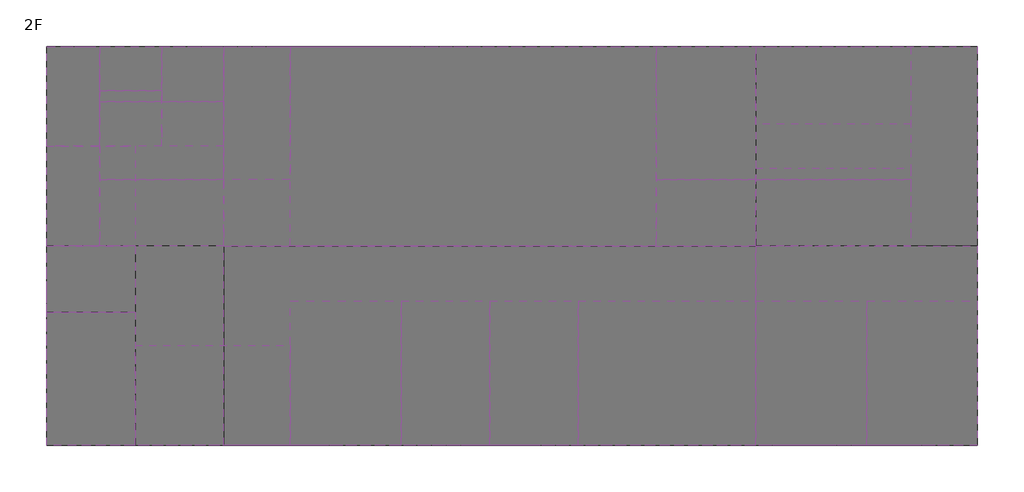
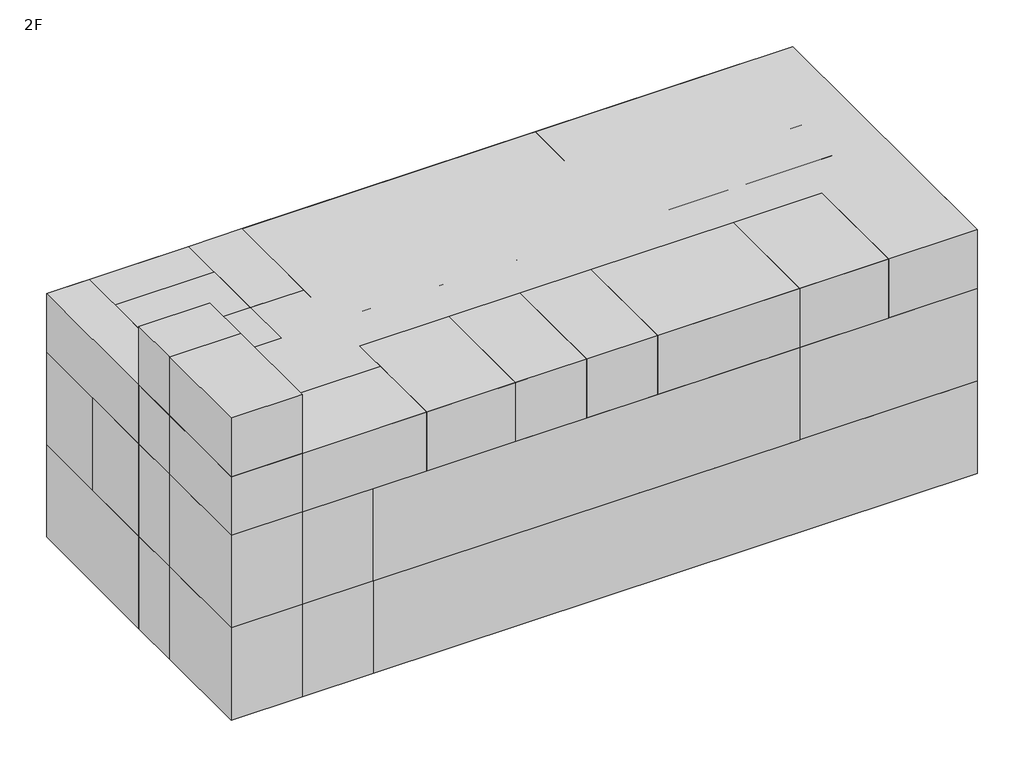
# One storey: 39 proxies.
# Revit data of these elements (continued)
# Room at (82459.652, 177423.861) mm, phase "New Construction", upper offset 2438.4 mm, lower offset 0 mm (continued)
#   Name = "Electrical Room (GIS)"
#   Interior Finish = "IW5..N/A..N/A,,WK1..N/A,,FL1,,CL1..N/A"
#   Exterior Finish = "N/A..N/A,,EW1..EW2..N/A"
# Room at (51459.652, 168423.861) mm, phase "New Construction", upper offset 2438.4 mm, lower offset 0 mm
#   Department = "AR"
#   Number = "2.3"
#   Name = "Lobby"
#   Interior Finish = "IW5..N/A..N/A,,WK3..N/A,,FL2,,CL3..N/A"
#   Exterior Finish = "N/A..N/A,,EW2..N/A..N/A"
# Room at (47459.652, 171423.861) mm, phase "New Construction", upper offset 2438.4 mm, lower offset 0 mm
#   Department = "PATHV2"
#   Number = "2.4"
#   Name = "Elevator"
#   Interior Finish = "N/A..N/A..N/A,,N/A..N/A,,,,N/A..N/A"
#   Exterior Finish = "N/A..N/A,,EW2..N/A..N/A"
# Room at (47459.652, 166923.861) mm, phase "New Construction", upper offset 2438.4 mm, lower offset 0 mm
#   Department = "PATHV1"
#   Number = "2.5"
#   Name = "Staircase"
#   Interior Finish = "IW5..N/A..N/A,,WK3..N/A,,FL2,,CL1..N/A"
#   Exterior Finish = "N/A..N/A,,EW2..N/A..N/A"
# Room at (65459.652, 177423.861) mm, phase "New Construction", upper offset 2438.4 mm, lower offset 0 mm
#   Department = "CI"
#   Number = "3.0"
#   Name = "Central Control Room"
#   Interior Finish = "IW5..N/A..N/A,,N/A..N/A,,FL5,,CL3..N/A"
#   Exterior Finish = "N/A..N/A,,EW1..N/A..N/A"
# Room at (65459.652, 168423.861) mm, phase "New Construction", upper offset 2438.4 mm, lower offset 0 mm
#   Department = "CI"
#   Number = "3.1"
#   Name = "Electronic Room"
#   Interior Finish = "IW5..N/A..N/A,,N/A..N/A,,FL5,,CL3..N/A"
#   Exterior Finish = "N/A..N/A,,EW1..N/A..N/A"
# Room at (80959.652, 180173.861) mm, phase "New Construction", upper offset 2438.4 mm, lower offset 0 mm
#   Department = "AR"
#   Number = "3.2"
#   Name = "Computer Room"
#   Interior Finish = "IW5..N/A..N/A,,N/A..N/A,,FL5,,CL3..N/A"
#   Exterior Finish = "N/A..N/A,,EW2..N/A..N/A"
# Room at (82459.652, 168423.861) mm, phase "New Construction", upper offset 2438.4 mm, lower offset 0 mm
#   Department = "EL"
#   Number = "3.3"
#   Name = "Electrical Room -3"
#   Interior Finish = "IW5..N/A..N/A,,N/A..N/A,,FL5,,CL3..N/A"
#   Exterior Finish = "N/A..N/A,,EW2..N/A..N/A"
# Room at (80959.652, 174673.861) mm, phase "New Construction", upper offset 2438.4 mm, lower offset 0 mm
#   Department = "CI"
#   Number = "3.4"
#   Name = "Communication Room"
#   Interior Finish = "IW5..N/A..N/A,,N/A..N/A,,FL5,,CL3..N/A"
#   Exterior Finish = "N/A..N/A,,N/A..N/A..N/A"
# Room at (46659.652, 179673.861) mm, phase "New Construction", upper offset 2438.4 mm, lower offset 0 mm
#   Department = "PATHV3"
#   Number = "3.5"
#   Name = "Duct Shaft"
#   Interior Finish = "N/A..N/A..N/A,,N/A..N/A,,,,N/A..N/A"
#   Exterior Finish = "N/A..N/A,,EW2..N/A..N/A"
# Room at (47459.652, 175173.861) mm, phase "New Construction", upper offset 2438.4 mm, lower offset 0 mm
#   Department = "AR"
#   Number = "3.6"
#   Name = "Toilet (M)"
#   Interior Finish = "IW3..N/A..N/A,,N/A..N/A,,FL3,,CL4..N/A"
#   Exterior Finish = "N/A..N/A,,EW2..N/A..N/A"
# Room at (52059.652, 179673.861) mm, phase "New Construction", upper offset 2438.4 mm, lower offset 0 mm
#   Department = "AR"
#   Number = "3.7"
#   Name = "Toilet"
#   Interior Finish = "IW3..N/A..N/A,,N/A..N/A,,FL3,,CL4..N/A"
#   Exterior Finish = "N/A..N/A,,EW2..N/A..N/A"
# Room at (49259.652, 180923.861) mm, phase "New Construction", upper offset 2438.4 mm, lower offset 0 mm
#   Department = "AR"
#   Number = "3.8"
#   Name = "Shower"
#   Interior Finish = "IW3..N/A..N/A,,N/A..N/A,,FL3,,CL4..N/A"
#   Exterior Finish = "N/A..N/A,,EW2..N/A..N/A"
# Room at (49259.652, 178673.861) mm, phase "New Construction", upper offset 2438.4 mm, lower offset 0 mm
#   Department = "AR"
#   Number = "3.9"
#   Name = "Locker(F)"
#   Interior Finish = "IW5..N/A..N/A,,WK3..N/A,,FL2,,CL3..N/A"
#   Exterior Finish = "N/A..N/A,,N/A..N/A..N/A"
# Room at (47459.652, 171423.861) mm, phase "New Construction", upper offset 2438.4 mm, lower offset 0 mm
#   Department = "PATHV2"
#   Number = "3.10"
#   Name = "Elevator"
#   Interior Finish = "N/A..N/A..N/A,,N/A..N/A,,,,N/A..N/A"
#   Exterior Finish = "N/A..N/A,,EW2..N/A..N/A"
# Room at (47459.652, 166923.861) mm, phase "New Construction", upper offset 2438.4 mm, lower offset 0 mm
#   Department = "PATHV1"
#   Number = "3.11"
#   Name = "Staircase"
#   Interior Finish = "IW5..N/A..N/A,,WK3..N/A,,FL2,,CL1..N/A"
#   Exterior Finish = "N/A..N/A,,EW2..N/A..N/A"
# Room at (82459.652, 177423.861) mm, phase "New Construction", upper offset 2438.4 mm, lower offset 0 mm
#   Department = "AR"
#   Number = "3.12"
#   Name = "Corridor"
#   Interior Finish = "IW5..N/A..N/A,,WK3..N/A,,FL2,,CL3..N/A"
#   Exterior Finish = "N/A..N/A,,EW2..N/A..N/A"
# Room at (51459.652, 170673.861) mm, phase "New Construction", upper offset 2438.4 mm, lower offset 0 mm
#   Department = "AR"
#   Number = "3.13"
#   Name = "Corridor"
#   Interior Finish = "IW5..N/A..N/A,,WK3..N/A,,FL2,,CL3..N/A"
#   Exterior Finish = "N/A..N/A,,EW2..N/A..N/A"
# Room at (63459.652, 167173.861) mm, phase "New Construction", upper offset 2438.4 mm, lower offset 0 mm
#   Department = "AR"
#   Number = "4.0"
#   Name = "Manager Office-1"
#   Interior Finish = "IW5..N/A..N/A,,WK3..N/A,,FL2,,CL3..N/A"
#   Exterior Finish = "RF1..N/A,,EW1..N/A..N/A"
# Room at (67459.652, 167173.861) mm, phase "New Construction", upper offset 2438.4 mm, lower offset 0 mm
#   Department = "AR"
#   Number = "4.1"
#   Name = "Manager Office-2"
#   Interior Finish = "IW5..N/A..N/A,,WK3..N/A,,FL2,,CL3..N/A"
#   Exterior Finish = "RF1..N/A,,EW1..N/A..N/A"
# Room at (78709.652, 178923.861) mm, phase "New Construction", upper offset 2438.4 mm, lower offset 0 mm
#   Department = "AR"
#   Number = "4.2"
#   Name = "Meeting Room-1"
#   Interior Finish = "IW5..N/A..N/A,,WK3..N/A,,FL2,,CL3..N/A"
#   Exterior Finish = "RF1..N/A,,EW1..EW2..N/A"
# Room at (73459.652, 167173.861) mm, phase "New Construction", upper offset 2438.4 mm, lower offset 0 mm
#   Department = "AR"
#   Number = "4.3"
#   Name = "Meeting Room-2"
#   Interior Finish = "IW5..N/A..N/A,,WK3..N/A,,FL2,,CL3..N/A"
#   Exterior Finish = "RF1..N/A,,EW1..N/A..N/A"
# Room at (64709.652, 177423.861) mm, phase "New Construction", upper offset 2438.4 mm, lower offset 0 mm
#   Department = "HV"
#   Number = "4.4"
#   Name = "Open Office"
#   Interior Finish = "IW5..N/A..N/A,,WK3..N/A,,FL2,,CL3..N/A"
#   Exterior Finish = "RF1..N/A,,EW1..N/A..N/A"
# Room at (79959.652, 167173.861) mm, phase "New Construction", upper offset 2438.4 mm, lower offset 0 mm
#   Department = "AR"
#   Number = "4.5"
#   Name = "Office-1"
#   Interior Finish = "IW5..N/A..N/A,,WK3..N/A,,FL2,,CL3..N/A"
#   Exterior Finish = "RF1..N/A,,EW2..N/A..N/A"
# Room at (84959.652, 167173.861) mm, phase "New Construction", upper offset 2438.4 mm, lower offset 0 mm
#   Department = "FF"
#   Number = "4.6"
#   Name = "Fire Gas Room"
#   Interior Finish = "IW5..N/A..N/A,,WK1..N/A,,FL1,,N/A..N/A"
#   Exterior Finish = "RF1..N/A,,EW2..N/A..N/A"
# Room at (78709.652, 174423.861) mm, phase "New Construction", upper offset 2438.4 mm, lower offset 0 mm
#   Department = "AR"
#   Number = "4.7"
#   Name = "Document Room"
#   Interior Finish = "IW5..N/A..N/A,,WK3..N/A,,FL2,,CL3..N/A"
#   Exterior Finish = "RF1..N/A,,N/A..N/A..N/A"
# Room at (58959.652, 167173.861) mm, phase "New Construction", upper offset 2438.4 mm, lower offset 0 mm
#   Department = "AR"
#   Number = "4.8"
#   Name = "Storage"
#   Interior Finish = "IW5..N/A..N/A,,WK3..N/A,,FL2,,CL3..N/A"
#   Exterior Finish = "RF1..N/A,,EW1..N/A..N/A"
# Room at (52959.652, 166173.861) mm, phase "New Construction", upper offset 2438.4 mm, lower offset 0 mm
#   Department = "AR"
#   Number = "4.9"
#   Name = "Break Room"
#   Interior Finish = "IW5..N/A..N/A,,WK3..N/A,,FL2,,CL3..N/A"
#   Exterior Finish = "RF1..N/A,,EW2..N/A..N/A"
# Room at (50659.652, 177673.861) mm, phase "New Construction", upper offset 2438.4 mm, lower offset 0 mm
#   Department = "AR"
#   Number = "4.10"
#   Name = "Toilet"
#   Interior Finish = "IW3..N/A..N/A,,N/A..N/A,,FL3,,CL4..N/A"
#   Exterior Finish = "RF1..N/A,,N/A..N/A..N/A"
# Room at (50659.652, 180673.861) mm, phase "New Construction", upper offset 2438.4 mm, lower offset 0 mm
#   Department = "AR"
#   Number = "4.11"
#   Name = "Shower"
#   Interior Finish = "IW3..N/A..N/A,,N/A..N/A,,FL3,,CL4..N/A"
#   Exterior Finish = "RF1..N/A,,EW2..N/A..N/A"
# Room at (54959.652, 178923.861) mm, phase "New Construction", upper offset 2438.4 mm, lower offset 0 mm
#   Department = "AR"
#   Number = "4.12"
#   Name = "Locker(M)"
#   Interior Finish = "IW5..N/A..N/A,,WK3..N/A,,FL2,,CL3..N/A"
#   Exterior Finish = "RF1..N/A,,EW1..N/A..N/A"
# Room at (50659.652, 174423.861) mm, phase "New Construction", upper offset 2438.4 mm, lower offset 0 mm
#   Department = "AR"
#   Number = "4.13"
#   Name = "Toilet(F)"
#   Interior Finish = "IW3..N/A..N/A,,N/A..N/A,,FL3,,CL4..N/A"
#   Exterior Finish = "RF1..N/A,,N/A..N/A..N/A"
# Room at (46659.652, 177423.861) mm, phase "New Construction", upper offset 2438.4 mm, lower offset 0 mm
#   Department = "PATHV3"
#   Number = "4.14"
#   Name = "Duct Shaft"
#   Interior Finish = "N/A..N/A..N/A,,N/A..N/A,,,,N/A..N/A"
#   Exterior Finish = "RF1..N/A,,EW2..N/A..N/A"
# Room at (47459.652, 171423.861) mm, phase "New Construction", upper offset 2438.4 mm, lower offset 0 mm
#   Department = "PATHV2"
#   Number = "4.15"
#   Name = "Elevator"
#   Interior Finish = "N/A..N/A..N/A,,N/A..N/A,,,,N/A..N/A"
#   Exterior Finish = "N/A..N/A,,EW2..N/A..N/A"
# Room at (47459.652, 166923.861) mm, phase "New Construction", upper offset 2438.4 mm, lower offset 0 mm
#   Department = "PATHV1"
#   Number = "4.16"
#   Name = "Staircase"
#   Interior Finish = "IW5..N/A..N/A,,N/A..N/A,,FL2,,CL1..N/A"
#   Exterior Finish = "N/A..N/A,,EW2..N/A..N/A"
# Room at (61397.694, 171673.861) mm, phase "New Construction", upper offset 2438.4 mm, lower offset 0 mm
#   Department = "AR"
#   Number = "4.17"
#   Name = "Corridor"
#   Interior Finish = "IW5..N/A..N/A,,WK3..N/A,,FL2,,CL3..N/A"
#   Exterior Finish = "RF1..N/A,,EW2..N/A..N/A"
# Room at (47459.652, 171423.861) mm, phase "New Construction", upper offset 2438.4 mm, lower offset 0 mm
#   Department = "PATHV2"
#   Number = "5.0"
#   Name = "Elevator"
#   Interior Finish = "N/A..N/A..N/A,,N/A..N/A,,,,N/A..N/A"
#   Exterior Finish = "RF1..N/A,,EW2..EW1..N/A"
# Room at (47459.652, 166923.861) mm, phase "New Construction", upper offset 2438.4 mm, lower offset 0 mm
#   Department = "PATHV1"
#   Number = "5.1"
#   Name = "Staircase"
#   Interior Finish = "IW5..N/A..N/A,,WK3..N/A,,FL2,,N/A..N/A"
#   Exterior Finish = "RF1..N/A,,EW2..EW1..N/A"
